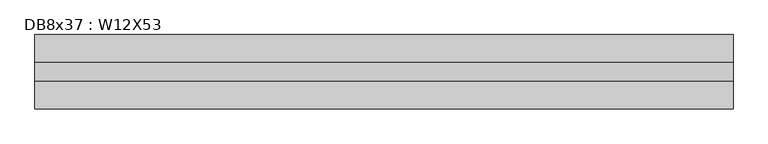
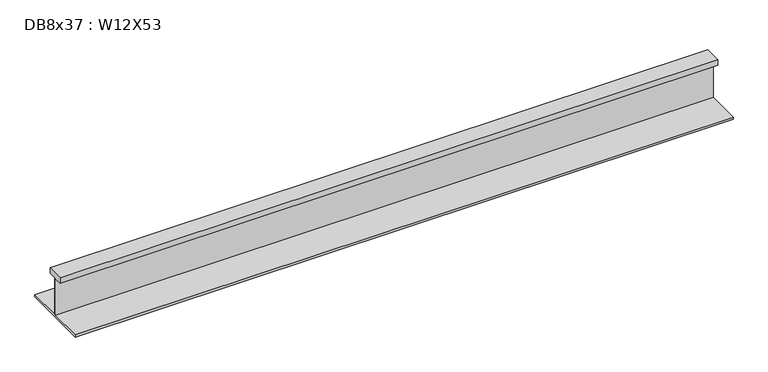
"""IFC4 building model written with IfcOpenShell, lengths in millimetres: beam geometry, DB8x37 : W12X53."""

from ifc_helpers import new_model, si_unit, frame, origin, place, context, project, spatial, polyline, outline, extrude, source, transform, mapped, element, save


def db8x37_w12x53_bd5c36fb(model_context):
    return source(origin(), model_context, "Body", "SweptSolid", [
        extrude(outline(polyline([(38.1, 145.415), (38.1, 120.015), (2.921, 120.015), (2.921, -48.4505), (152.4, -48.4505), (152.4, -58.1025), (-152.4, -58.1025), (-152.4, -48.4505), (-2.921, -48.4505), (-2.921, 120.015), (-38.1, 120.015), (-38.1, 145.415), (38.1, 145.415)])), frame((-1428.1780856, 0.0, 0.0), z_axis=(1.0, 0.0, 0.0), x_axis=(0.0, 1.0, 0.0)), (0.0, 0.0, 1.0), 2866.3907891),
    ])


if __name__ == "__main__":
    model = new_model("IFC4")
    model_context = context("Model", 3, world=origin())
    ifc_project = project(units=[si_unit("LENGTHUNIT", "METRE", prefix="MILLI")], contexts=[model_context])
    site = spatial("IfcSite", under=ifc_project)
    building = spatial("IfcBuilding", under=site)
    placement = place(None, origin())
    db8x37_w12x53_shape = db8x37_w12x53_bd5c36fb(model_context)
    element("IfcBeam", 1, ObjectType="DB8x37 : W12X53", at=placement, inside=building, context=model_context, shape_type="MappedRepresentation", body=[
        mapped(db8x37_w12x53_shape, transform((0.0, 0.0, 0.0), x_axis=(1.0, 0.0, 0.0), y_axis=(0.0, 1.0, 0.0), z_axis=(0.0, 0.0, 1.0))),
    ])
    save(model, "model.ifc")

# Revit data of these elements
# Type "DB8x37 : W12X53"
#   Assembly Code = "B10"
#   W = 53
#   Length [instance default] = 5' - 0"
#   bf = 0' - 10"
#   d = 1' - 0.1"
#   k = 0' - 1 3/8"
#   k2 = 0' - 0.8"
#   tf = 0' - 0.575"
#   tw = 0' - 0.345"
#   A = 0.108333 SF
#   Structural Material [instance default] = Steel ASTM A992
# Element 1 (IfcBeam, "DB8x37 : W12X53")
#   Materials on its faces: "Steel ASTM A992"
# Materials
#   "Steel ASTM A992": class "Metal", colour RGB 199 199 199, transparency 0, Description = "Structural steel 50ksi", Cost = 0
